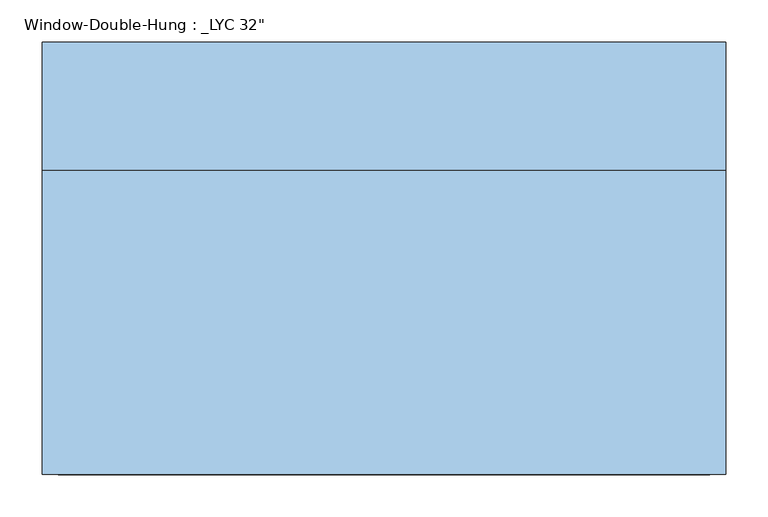
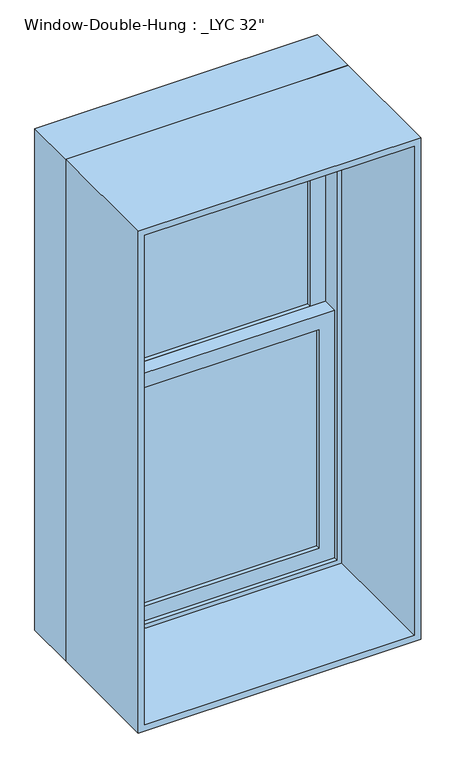
"""IFC4 building model written with IfcOpenShell, lengths in millimetres: window geometry."""

from ifc_helpers import new_model, si_unit, frame, origin, place, context, project, spatial, polyline, outline, extrude, source, transform, mapped, element, save


def window_2aac4284(model_context):
    return source(origin(), model_context, "Body", "SweptSolid", [
        extrude(outline(polyline([(330.2, 158.75), (330.2, 152.4), (-330.2, 152.4), (-330.2, 158.75), (330.2, 158.75)])), frame((0.0, 0.0, 990.6), z_axis=(0.0, 0.0, 1.0), x_axis=(1.0, 0.0, 0.0)), (0.0, 0.0, 1.0), 663.575),
        extrude(outline(polyline([(-330.2, 146.05), (330.2, 146.05), (330.2, 139.7), (-330.2, 139.7), (-330.2, 146.05)])), frame((0.0, 0.0, 990.6), z_axis=(0.0, 0.0, 1.0), x_axis=(1.0, 0.0, 0.0)), (0.0, 0.0, 1.0), 663.575),
        extrude(outline(polyline([(330.2, 203.2), (330.2, 196.85), (-330.2, 196.85), (-330.2, 203.2), (330.2, 203.2)])), frame((0.0, 0.0, 1698.625), z_axis=(0.0, 0.0, 1.0), x_axis=(1.0, 0.0, 0.0)), (0.0, 0.0, 1.0), 663.575),
        extrude(outline(polyline([(-330.2, 190.5), (330.2, 190.5), (330.2, 184.15), (-330.2, 184.15), (-330.2, 190.5)])), frame((0.0, 0.0, 1698.625), z_axis=(0.0, 0.0, 1.0), x_axis=(1.0, 0.0, 0.0)), (0.0, 0.0, 1.0), 663.575),
        extrude(outline(polyline([(1698.625, -374.65), (946.15, -374.65), (946.15, 374.65), (1698.625, 374.65), (1698.625, -374.65)]), holes=[polyline([(1654.175, 330.2), (990.6, 330.2), (990.6, -330.2), (1654.175, -330.2), (1654.175, 330.2)])]), frame((0.0, 127.0, 0.0), z_axis=(0.0, 1.0, 0.0), x_axis=(0.0, 0.0, 1.0)), (0.0, 0.0, 1.0), 44.45),
        extrude(outline(polyline([(2406.65, -374.65), (1654.175, -374.65), (1654.175, 374.65), (2406.65, 374.65), (2406.65, -374.65)]), holes=[polyline([(2362.2, 330.2), (1698.625, 330.2), (1698.625, -330.2), (2362.2, -330.2), (2362.2, 330.2)])]), frame((0.0, 171.45, 0.0), z_axis=(0.0, 1.0, 0.0), x_axis=(0.0, 0.0, 1.0)), (0.0, 0.0, 1.0), 44.45),
        extrude(outline(polyline([(2438.4, -406.4), (914.4, -406.4), (914.4, 406.4), (2438.4, 406.4), (2438.4, -406.4)]), holes=[polyline([(2406.65, 374.65), (946.15, 374.65), (946.15, -374.65), (2406.65, -374.65), (2406.65, 374.65)])]), frame((0.0, 114.3, 0.0), z_axis=(0.0, 1.0, 0.0), x_axis=(0.0, 0.0, 1.0)), (0.0, 0.0, 1.0), 152.4),
        extrude(outline(polyline([(2438.4, 406.4), (2438.4, -406.4), (914.4, -406.4), (914.4, 406.4), (2438.4, 406.4)]), holes=[polyline([(2419.35, 387.35), (933.45, 387.35), (933.45, -387.35), (2419.35, -387.35), (2419.35, 387.35)])]), frame((0.0, -247.65, 0.0), z_axis=(0.0, 1.0, 0.0), x_axis=(0.0, 0.0, 1.0)), (0.0, 0.0, 1.0), 361.95),
    ])


if __name__ == "__main__":
    model = new_model("IFC4")
    model_context = context("Model", 3, world=origin())
    ifc_project = project(units=[si_unit("LENGTHUNIT", "METRE", prefix="MILLI")], contexts=[model_context])
    site = spatial("IfcSite", under=ifc_project)
    building = spatial("IfcBuilding", under=site)
    placement = place(None, origin())
    window_shape = window_2aac4284(model_context)
    element("IfcWindow", 1, ObjectType="Window-Double-Hung : _LYC 32\"", at=placement, inside=building, context=model_context, shape_type="MappedRepresentation", body=[
        mapped(window_shape, transform((0.0, 0.0, 0.0), x_axis=(1.0, 0.0, 0.0), y_axis=(0.0, 1.0, 0.0), z_axis=(0.0, 0.0, 1.0))),
    ])
    save(model, "model.ifc")

# Revit data of these elements
# Type "Window-Double-Hung : _LYC 32\""
#   Type Mark = "25"
#   Fire Rating = "0.5h"
#   Assembly Code = "B2020100"
#   Wall Thickness [instance default] = 0' - 6"
#   Visual Light Transmittance = 0.9
#   Thermal Resistance (R) = 1.8146 (h·ft²·°F)/BTU
#   Solar Heat Gain Coefficient = 0.78
#   Rough Width = 2' - 8 1/2"
#   Rough Height = 5' - 0 1/2"
#   Muntin Width = 2' - 2"
#   Muntin Height = 2' - 2 1/8"
#   Interior Wall Closure [instance default] = 0' - 1 1/2"
#   Heat Transfer Coefficient (U) = 0.6496 BTU/(h·ft²·°F)
#   Frame Extension [instance default] = 0' - 2"
#   Exterior Wall Closure [instance default] = 0' - 0 1/2"
#   Extension Jamb [instance default] = 0' - 0 3/4"
#   Height = 5' - 0"
#   Width = 2' - 8"
#   Window Inset [instance default] = 0' - 0 3/4"
#   Top Muntin Visibility = yes
#   Interior Trim Visibility [instance default] = yes
#   Indicator Visibility [instance default] = yes
#   Exterior Trim Visibility [instance default] = yes
#   Extension Jamb Visibility [instance default] = yes
#   Define Thermal Properties by = 1
#   Bottom Muntin Visibility = yes
#   Muntin Pattern = Muntin Pattern_2x2 : Muntin Pattern_2x2
#   Interior Trim Material = Wood - Stained
#   Interior Trim = Trim-Window-Interior-Flat : Picture Frame
#   Interior Frame Material = Wood - Stained
#   Glass Panel Material = Glass
#   Exterior Trim Material = Clad - White
#   Exterior Trim = Trim-Window-Exterior-Flat : with Sill
#   Exterior Frame Material = Clad - White
#   Construction Type Id = ""
#   Wall Closure = (empty or 0)
#   Analytic Construction = (empty or 0)
# Element 1 (IfcWindow, "Window-Double-Hung : _LYC 32\"")
#   Wall Thickness = 1' - 7 1/2"
#   Extension Jamb = 1' - 2 1/4"
#   Materials on its faces: "Wood - Stained", "Glass", "Clad - White"
# Materials
#   "Wood - Stained": class "Wood", colour RGB 224 178 126, transparency 0, Cost = 0
#   "Glass": class "Unassigned", colour RGB 0 128 192, transparency 0.75
#   "Clad - White": class "Wood", colour RGB 242 242 238, transparency 0, Cost = 0
